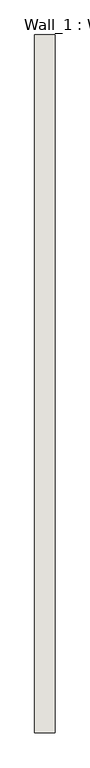
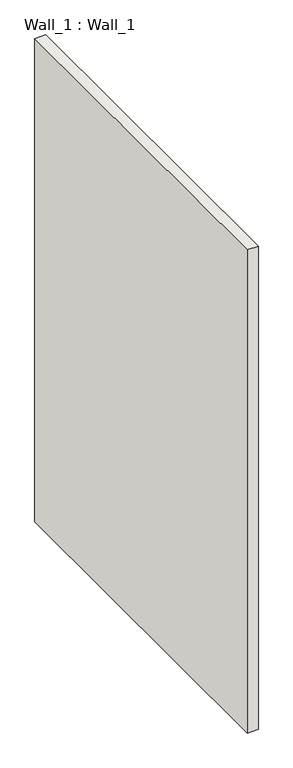
"""IFC4 building model written with IfcOpenShell, lengths in millimetres: wall geometry, Wall_1 : Wall_1."""

from ifc_helpers import new_model, si_unit, origin, origin_with_axes, place, context, project, spatial, polyline, outline, extrude, source, transform, mapped, element, save


def wall_1_wall_1_841e26ce(model_context):
    return source(origin(), model_context, "Body", "SweptSolid", [
        extrude(outline(polyline([(100.0, 3770.0), (100.0, 380.0), (0.0, 380.0), (0.0, 3770.0), (100.0, 3770.0)])), origin_with_axes(), (0.0, 0.0, 1.0), 4700.0),
    ])


if __name__ == "__main__":
    model = new_model("IFC4")
    model_context = context("Model", 3, world=origin())
    ifc_project = project(units=[si_unit("LENGTHUNIT", "METRE", prefix="MILLI")], contexts=[model_context])
    site = spatial("IfcSite", under=ifc_project)
    building = spatial("IfcBuilding", under=site)
    placement = place(None, origin())
    wall_1_wall_1_shape = wall_1_wall_1_841e26ce(model_context)
    element("IfcWall", 1, ObjectType="Wall_1 : Wall_1", at=placement, inside=building, context=model_context, shape_type="MappedRepresentation", body=[
        mapped(wall_1_wall_1_shape, transform((0.0, 0.0, 0.0), x_axis=(1.0, 0.0, 0.0), y_axis=(0.0, 1.0, 0.0), z_axis=(0.0, 0.0, 1.0))),
    ])
    save(model, "model.ifc")

# Revit data of these elements
# Type "Wall_1 : Wall_1"
#   NameOverride = "Wall_1"
# Element 1 (IfcWall, "Wall_1 : Wall_1")
#   Materials on its faces: "IfcSurfaceStyle #33"
# Materials
#   "IfcSurfaceStyle #33": class "Unassigned", colour RGB 214 214 214, transparency 0
